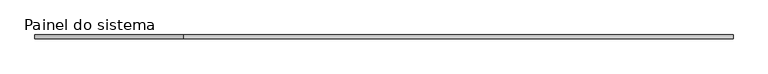
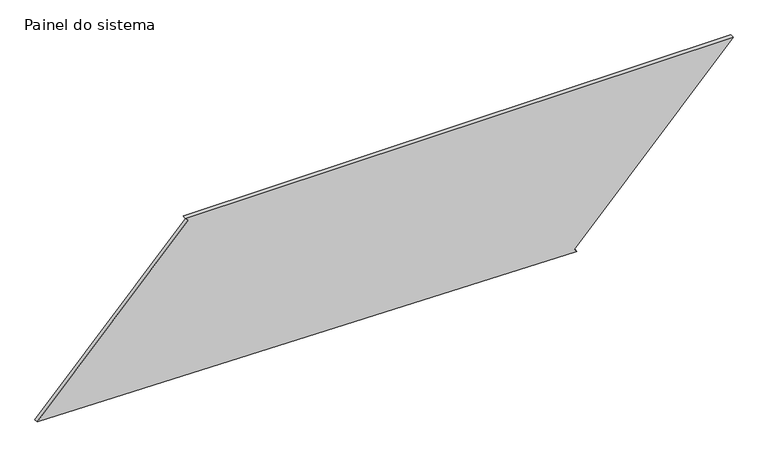
"""IFC4 building model written with IfcOpenShell, lengths in millimetres: plate geometry, Painel do sistema : Envidraçado."""

from ifc_helpers import new_model, si_unit, frame, origin, place, context, project, spatial, polyline, outline, extrude, source, transform, mapped, element, save


def painel_do_sistema_55dbc004(model_context):
    return source(origin(), model_context, "Body", "SweptSolid", [
        extrude(outline(polyline([(0.0, 1224.1615648), (17.1196584, 1205.9429673), (1097.7039086, 2221.3467685), (1097.7039086, -1274.5712488), (1080.5842503, -1256.3526512), (53.6455649, -2221.3467685), (0.0, 1224.1615648)])), frame((0.0, 24.5, 0.0), z_axis=(0.0, 1.0, 0.0), x_axis=(0.0, 0.0, 1.0)), (0.0, 0.0, 1.0), 25.0),
    ])


if __name__ == "__main__":
    model = new_model("IFC4")
    model_context = context("Model", 3, world=origin())
    ifc_project = project(units=[si_unit("LENGTHUNIT", "METRE", prefix="MILLI")], contexts=[model_context])
    site = spatial("IfcSite", under=ifc_project)
    building = spatial("IfcBuilding", under=site)
    placement = place(None, origin())
    painel_do_sistema_shape = painel_do_sistema_55dbc004(model_context)
    element("IfcPlate", 1, ObjectType="Painel do sistema : Envidraçado", at=placement, inside=building, context=model_context, shape_type="MappedRepresentation", body=[
        mapped(painel_do_sistema_shape, transform((0.0, 0.0, 0.0), x_axis=(1.0, 0.0, 0.0), y_axis=(0.0, 1.0, 0.0), z_axis=(0.0, 0.0, 1.0))),
    ])
    save(model, "model.ifc")

# Revit data of these elements
# Type "Painel do sistema : Envidraçado"
#   Construction Type Id = "GSP4R"
#   Analytic Construction = "Vidraça única Pilkington 1/8 pol"
#   Visual Light Transmittance = 0.9
#   Solar Heat Gain Coefficient = 0.86
#   Heat Transfer Coefficient (U) = 6.7069 W/(m²·K)
# Element 1 (IfcPlate, "Painel do sistema : Envidraçado")
#   Materials on its faces: "Vidro"
# Materials
#   "Vidro": class "Vidro", colour RGB 0 128 192, transparency 0.9, Description = "Vidro de sílica", Cost = 0
